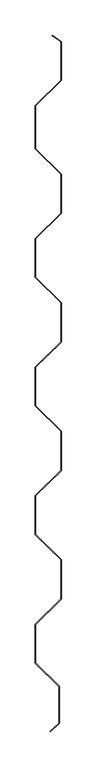
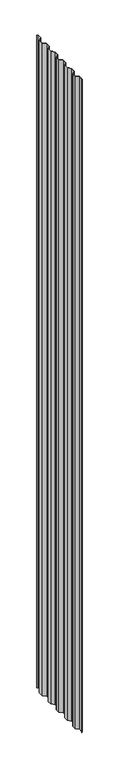
"""IFC4 building model written with IfcOpenShell, lengths in millimetres: proxy geometry, Generic Models 2:Generic Models 2:310765:Generic Models 2:310765 : Generic Models 2:Generic Models 2:310765:8 : Generic Models 2:Generic Models 2:310765:Generic Models 2:310765 : Generic Models 2:Generic Models 2:310765:300385."""

from ifc_helpers import new_model, si_unit, origin, origin_with_axes, place, context, project, spatial, polyline, outline, extrude, source, transform, mapped, element, save


def generic_models_4c549ba2(model_context):
    return source(origin(), model_context, "Body", "SweptSolid", [
        extrude(outline(polyline([(756171.5135611, -578737.8387429), (756158.4054901, -578749.6944892), (756157.8435183, -578749.1325174), (756170.7198111, -578737.4864055), (756170.7198111, -578685.5800515), (756136.1617239, -578651.9480667), (756136.1617239, -578596.7685069), (756173.4679739, -578560.6063152), (756173.4679739, -578505.2311896), (756136.1617239, -578469.0689979), (756136.1617239, -578413.8885069), (756173.4679739, -578377.7263152), (756173.4679739, -578322.3511896), (756136.1617239, -578286.1889979), (756136.1617239, -578231.0085069), (756173.4679739, -578194.8463152), (756173.4679739, -578139.4711896), (756136.1617239, -578103.3089979), (756136.1617239, -578048.1285069), (756173.4679739, -578011.9663152), (756173.4679739, -577956.5911896), (756136.1617239, -577920.4289979), (756136.1617239, -577858.8985069), (756173.4679739, -577822.7363152), (756173.4679739, -577768.2077525), (756160.6983766, -577759.2663842), (756161.1536529, -577758.6161822), (756174.2617239, -577767.7945524), (756174.2617239, -577823.0723607), (756136.9554739, -577859.2345524), (756136.9554739, -577920.0929524), (756174.2617239, -577956.255144), (756174.2617239, -578012.3023607), (756136.9554739, -578048.4645524), (756136.9554739, -578102.9729524), (756174.2617239, -578139.135144), (756174.2617239, -578195.1823607), (756136.9554739, -578231.3445524), (756136.9554739, -578285.8529524), (756174.2617239, -578322.015144), (756174.2617239, -578378.0623607), (756136.9554739, -578414.2245524), (756136.9554739, -578468.7329524), (756174.2617239, -578504.895144), (756174.2617239, -578560.9423607), (756136.9554739, -578597.1045524), (756136.9554739, -578651.6129524), (756171.5135611, -578685.2449371), (756171.5135611, -578737.8387429)])), origin_with_axes(), (0.0, 0.0, 1.0), 8788.3280821),
    ])


if __name__ == "__main__":
    model = new_model("IFC4")
    model_context = context("Model", 3, world=origin())
    ifc_project = project(units=[si_unit("LENGTHUNIT", "METRE", prefix="MILLI")], contexts=[model_context])
    site = spatial("IfcSite", under=ifc_project)
    building = spatial("IfcBuilding", under=site)
    placement = place(None, origin())
    generic_models_shape = generic_models_4c549ba2(model_context)
    element("IfcBuildingElementProxy", 1, Name="Generic Models 2:Generic Models 2:310765:Generic Models 2:310765 : Generic Models 2:Generic Models 2:310765:8 : Generic Models 2:Generic Models 2:310765:Generic Models 2:310765 : Generic Models 2:Generic Models 2:310765:300385", ObjectType="Generic Models 2:Generic Models 2:310765:Generic Models 2:310765 : Generic Models 2:Generic Models 2:310765:8 : Generic Models 2:Generic Models 2:310765:Generic Models 2:310765 : Generic Models 2:Generic Models 2:310765:300385", at=placement, inside=building, context=model_context, shape_type="MappedRepresentation", body=[
        mapped(generic_models_shape, transform((0.0, 0.0, 0.0), x_axis=(1.0, 0.0, 0.0), y_axis=(0.0, 1.0, 0.0), z_axis=(0.0, 0.0, 1.0))),
    ])
    save(model, "model.ifc")

# Revit data of these elements
# Type "Generic Models 2:Generic Models 2:310765:Generic Models 2:310765 : Generic Models 2:Generic Models 2:310765:8 : Generic Models 2:Generic Models 2:310765:Generic Models 2:310765 : Generic Models 2:Generic Models 2:310765:300385"
#   NameOverride = "Generic Models 2:Generic Models 2:310765:Generic Models 2:310765 : Generic Models 2:Generic Models 2:310765:300385"
#   ObjectTypeOverride = "Generic Models 2:310765 : Generic Models 2:Generic Models 2:310765"
#   Reference = "Generic Models 2"
#   Tag = "300385"
# Element 1 (IfcBuildingElementProxy, "Generic Models 2:Generic Models 2:310765:Generic Models 2:310765 : Generic Models 2:Generic Models 2:310765:8 : Generic Models 2:Generic Models 2:310765:Generic Models 2:310765 : Generic Models 2:Generic Models 2:310765:300385")
#   Materials on its faces: "VERTICAL CORRUGATED METAL PANEL - EXPOSED FASTENERS - (MBCI 7.2 PANEL)"
# Materials
#   "VERTICAL CORRUGATED METAL PANEL - EXPOSED FASTENERS - (MBCI 7.2 PANEL)": class "Generic", colour RGB 120 120 120, transparency 0, Cost = 0
